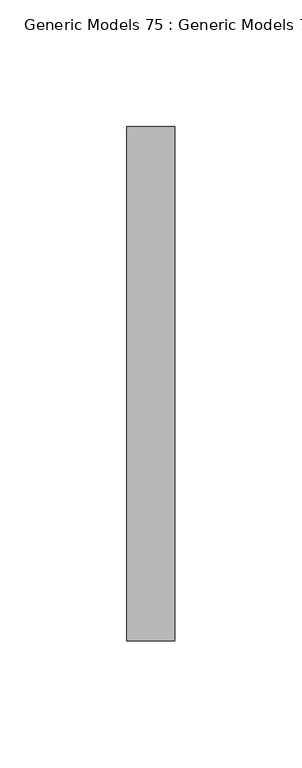
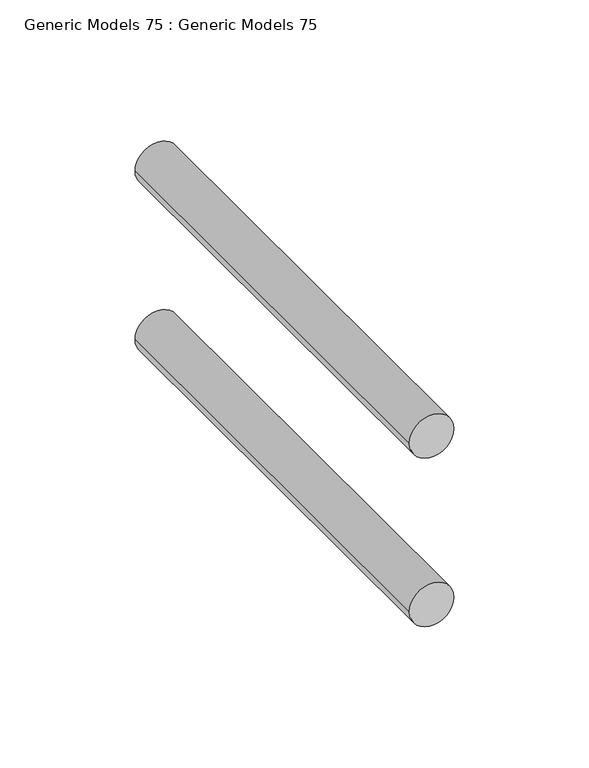
"""IFC4 building model written with IfcOpenShell, lengths in millimetres: proxy geometry, Generic Models 75 : Generic Models 75."""

from ifc_helpers import new_model, si_unit, point, frame, frame_2d, origin, place, context, project, spatial, circle_curve, trimmed, segment, composite_curve, outline, extrude, source, transform, mapped, element, save


def generic_models_75_generic_models_75_1193d190(model_context):
    return source(origin(), model_context, "Body", "SweptSolid", [
        extrude(outline(composite_curve([segment(trimmed(circle_curve(frame_2d((271559.3375, 31975.4096032)), 9.525), [point((271559.3375, 31965.8846032))], [point((271559.3375, 31984.9346032))], False, "CARTESIAN"), True, "CONTINUOUS"), segment(trimmed(circle_curve(frame_2d((271559.3375, 31975.4096032)), 9.525), [point((271559.3375, 31984.9346032))], [point((271559.3375, 31965.8846032))], False, "CARTESIAN"), True, "CONTINUOUS")], self_intersect=False)), frame((0.0, 30672.7406612, 0.0), z_axis=(0.0, 1.0, 0.0), x_axis=(0.0, 0.0, 1.0)), (0.0, 0.0, 1.0), 203.2),
        extrude(outline(composite_curve([segment(trimmed(circle_curve(frame_2d((271635.5375, 31975.4096032)), 9.525), [point((271635.5375, 31965.8846032))], [point((271635.5375, 31984.9346032))], False, "CARTESIAN"), True, "CONTINUOUS"), segment(trimmed(circle_curve(frame_2d((271635.5375, 31975.4096032)), 9.525), [point((271635.5375, 31984.9346032))], [point((271635.5375, 31965.8846032))], False, "CARTESIAN"), True, "CONTINUOUS")], self_intersect=False)), frame((0.0, 30672.7406612, 0.0), z_axis=(0.0, 1.0, 0.0), x_axis=(0.0, 0.0, 1.0)), (0.0, 0.0, 1.0), 203.2),
    ])


if __name__ == "__main__":
    model = new_model("IFC4")
    model_context = context("Model", 3, world=origin())
    ifc_project = project(units=[si_unit("LENGTHUNIT", "METRE", prefix="MILLI")], contexts=[model_context])
    site = spatial("IfcSite", under=ifc_project)
    building = spatial("IfcBuilding", under=site)
    placement = place(None, origin())
    generic_models_75_generic_models_75_shape = generic_models_75_generic_models_75_1193d190(model_context)
    element("IfcBuildingElementProxy", 1, Name="Generic Models 75 : Generic Models 75", ObjectType="Generic Models 75 : Generic Models 75", at=placement, inside=building, context=model_context, shape_type="MappedRepresentation", body=[
        mapped(generic_models_75_generic_models_75_shape, transform((0.0, 0.0, 0.0), x_axis=(1.0, 0.0, 0.0), y_axis=(0.0, 1.0, 0.0), z_axis=(0.0, 0.0, 1.0))),
    ])
    save(model, "model.ifc")
